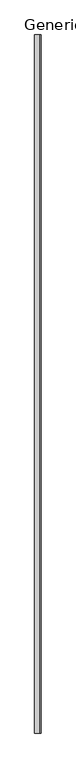
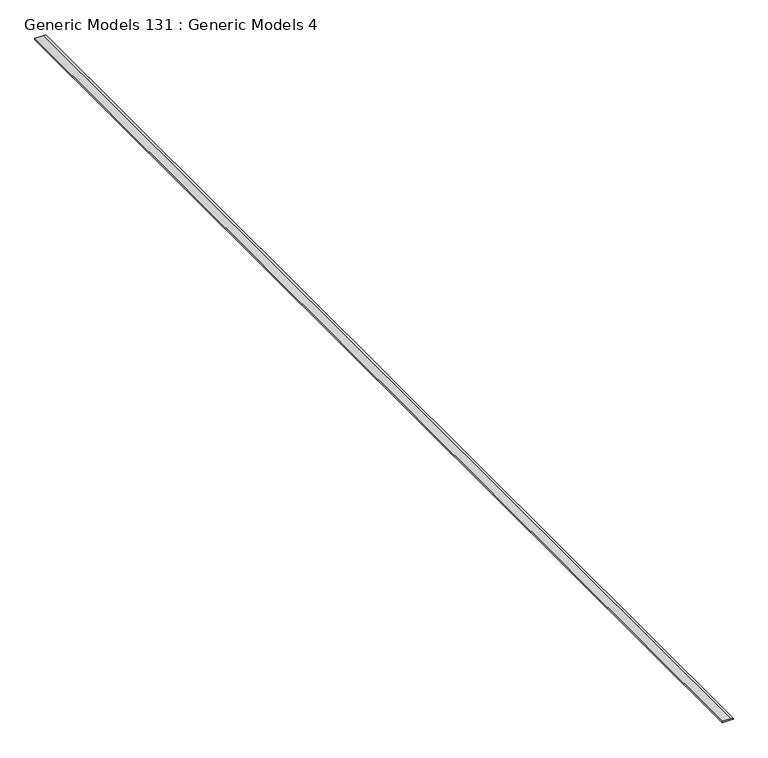
"""IFC4 building model written with IfcOpenShell, lengths in millimetres: proxy geometry, Generic Models 131 : Generic Models 4."""

import ifcopenshell
import ifcopenshell.guid

model = None  # the IFC model being written
_history = None  # IfcOwnerHistory: only IFC2X3 demands one
_inside = {}  # id of a spatial element -> (the spatial element, [elements in it])
_under = {}  # id of a project, library or spatial element -> (it, [spatial elements below it])
_declared = {}  # id of a project -> (the project, [libraries it declares])
_typed = {}  # id of a type object -> (the type object, [elements of that type])
_made_of = {}  # id of a material, layer set ... -> (it, [elements and type objects made of it])


def new_model(schema):
    """Start an empty IFC model of exactly this schema.

    Asked for "IFC4X3", IfcOpenShell would pick the latest addendum, in which some entities
    have other attributes; the version numbers below select the first issue.
    IFC2X3 requires an IfcOwnerHistory on every rooted entity: one is made here for all.
    """
    global model, _history
    if schema == "IFC4X3":
        model = ifcopenshell.file(schema_version=(4, 3, 0, 0))
    else:
        model = ifcopenshell.file(schema=schema)
    _inside.clear()
    _under.clear()
    _declared.clear()
    _typed.clear()
    _made_of.clear()
    _history = None
    if model.schema == "IFC2X3":
        org = make("IfcOrganization", Name="unknown")
        user = make(
            "IfcPersonAndOrganization",
            ThePerson=make("IfcPerson", FamilyName="unknown"),
            TheOrganization=org,
        )
        app = make(
            "IfcApplication",
            ApplicationDeveloper=org,
            Version="unknown",
            ApplicationFullName="unknown",
            ApplicationIdentifier="unknown",
        )
        _history = make(
            "IfcOwnerHistory",
            OwningUser=user,
            OwningApplication=app,
            ChangeAction="ADDED",
            CreationDate=0,
        )
    return model


def make(cls, **values):
    """One entity of the class cls with the attributes given. An attribute that is None is left unset."""
    return model.create_entity(
        cls, **{name: value for name, value in values.items() if value is not None}
    )


def rooted(cls, **values):
    """An entity with a GlobalId (a new one), such as an element, a storey or a relation."""
    return make(cls, GlobalId=ifcopenshell.guid.new(), OwnerHistory=_history, **values)


def si_unit(unit_type, name, prefix=None):
    """IfcSIUnit, for example si_unit("LENGTHUNIT", "METRE", prefix="MILLI")."""
    return make("IfcSIUnit", UnitType=unit_type, Prefix=prefix, Name=name)


def assignment(units):
    """IfcUnitAssignment: the units of a project."""
    return None if units is None else make("IfcUnitAssignment", Units=units)


def point(xyz):
    """IfcCartesianPoint."""
    return None if xyz is None else make("IfcCartesianPoint", Coordinates=xyz)


def direction(xyz):
    """IfcDirection."""
    return None if xyz is None else make("IfcDirection", DirectionRatios=xyz)


def frame(location, z_axis=None, x_axis=None):
    """IfcAxis2Placement3D, a coordinate frame: its origin and axes. An axis left out is left unset."""
    return make(
        "IfcAxis2Placement3D",
        Location=point(location),
        Axis=direction(z_axis),
        RefDirection=direction(x_axis),
    )


def origin():
    """The frame at (0, 0, 0) with its axes left unset."""
    return frame((0.0, 0.0, 0.0))


def place(relative_to, where):
    """IfcLocalPlacement: puts the frame where relative to a parent placement (None: the world)."""
    return make(
        "IfcLocalPlacement", PlacementRelTo=relative_to, RelativePlacement=where
    )


def context(
    kind, dimensions, precision=None, world=None, true_north=None, identifier=None
):
    """IfcGeometricRepresentationContext, for example the 3D "Model" context."""
    return make(
        "IfcGeometricRepresentationContext",
        ContextIdentifier=identifier,
        ContextType=kind,
        CoordinateSpaceDimension=dimensions,
        Precision=precision,
        WorldCoordinateSystem=world,
        TrueNorth=true_north,
    )


def project(units=None, contexts=None):
    """IfcProject with its units and contexts."""
    return rooted(
        "IfcProject",
        Name="project",
        RepresentationContexts=contexts,
        UnitsInContext=assignment(units),
    )


def spatial(cls, under=None, at=None, **own):
    """A site, building, storey or space (cls), placed at a placement, below another one or the project."""
    s = rooted(cls, ObjectPlacement=at, **own)
    if under is not None:
        _under.setdefault(under.id(), (under, []))[1].append(s)
    return s


def faces_of(points, faces, orient=None, outer=None):
    """IfcFace entities. A face is a list of loops; a loop is a list of indices into points, from 0.

    orient and outer hold one flag for each loop. By default every Orientation is true, the
    first loop of a face is its IfcFaceOuterBound and the others are IfcFaceBound.
    """
    made = []
    for i, loops in enumerate(faces):
        bounds = []
        for j, loop in enumerate(loops):
            is_outer = j == 0 if outer is None else outer[i][j]
            bounds.append(
                make(
                    "IfcFaceOuterBound" if is_outer else "IfcFaceBound",
                    Bound=make("IfcPolyLoop", Polygon=[points[k] for k in loop]),
                    Orientation=True if orient is None else orient[i][j],
                )
            )
        made.append(make("IfcFace", Bounds=bounds))
    return made


def faceted_brep(points, faces, orient=None, outer=None, voids=None):
    """IfcFacetedBrep: a solid bounded by flat faces; with voids (closed shells), ...WithVoids."""
    shared = [point(p) for p in points]
    hull = make("IfcClosedShell", CfsFaces=faces_of(shared, faces, orient, outer))
    if voids is None:
        return make("IfcFacetedBrep", Outer=hull)
    return make(
        "IfcFacetedBrepWithVoids",
        Outer=hull,
        Voids=[
            make(cls, CfsFaces=faces_of(shared, fs, o, b)) for cls, fs, o, b in voids
        ],
    )


def shape(context_of_items, identifier, shape_type, items):
    """IfcShapeRepresentation: the items that make up one representation, for example the "Body"."""
    return make(
        "IfcShapeRepresentation",
        ContextOfItems=context_of_items,
        RepresentationIdentifier=identifier,
        RepresentationType=shape_type,
        Items=items,
    )


def source(mapping_origin, context_of_items, identifier, shape_type, items):
    """IfcRepresentationMap: a shape defined once, which mapped items show again and again."""
    return make(
        "IfcRepresentationMap",
        MappingOrigin=mapping_origin,
        MappedRepresentation=shape(context_of_items, identifier, shape_type, items),
    )


def transform(
    local_origin,
    x_axis=None,
    y_axis=None,
    z_axis=None,
    scale=None,
    scale2=None,
    scale3=None,
    uniform=True,
):
    """IfcCartesianTransformationOperator3D, or its non-uniform kind. x_axis, y_axis, z_axis: its Axis1, 2, 3."""
    if uniform:
        return make(
            "IfcCartesianTransformationOperator3D",
            Axis1=direction(x_axis),
            Axis2=direction(y_axis),
            LocalOrigin=point(local_origin),
            Scale=scale,
            Axis3=direction(z_axis),
        )
    return make(
        "IfcCartesianTransformationOperator3DnonUniform",
        Axis1=direction(x_axis),
        Axis2=direction(y_axis),
        LocalOrigin=point(local_origin),
        Scale=scale,
        Axis3=direction(z_axis),
        Scale2=scale2,
        Scale3=scale3,
    )


def mapped(mapping_source, mapping_target):
    """IfcMappedItem: shows the shape of a source again, moved by a transform."""
    return make(
        "IfcMappedItem", MappingSource=mapping_source, MappingTarget=mapping_target
    )


def made_of(thing, what):
    """Note that an element or type object is made of a material, layer set ...; save() writes the relation."""
    if what is not None:
        _made_of.setdefault(what.id(), (what, []))[1].append(thing)
    return thing


def element(
    cls,
    number,
    at=None,
    inside=None,
    cuts=None,
    type_object=None,
    material=None,
    context=None,
    identifier="Body",
    shape_type=None,
    held_by="IfcProductDefinitionShape",
    body=None,
    shapes=None,
    **own,
):
    """One element of the class cls, such as IfcWall. Its Tag is "e" and its number.

    at: its placement. inside: the storey or other place that contains it. cuts: it is an
    opening in that element (IfcRelVoidsElement). A single representation is given by context,
    identifier, shape_type and body (its items); several are given by shapes. held_by: the class
    of the entity that holds the representations. save() writes the other relations.
    """
    e = rooted(cls, Tag="e%d" % number, ObjectPlacement=at, **own)
    if body is not None:
        shapes = [shape(context, identifier, shape_type, body)]
    if shapes is not None:
        e.Representation = make(held_by, Representations=shapes)
    if inside is not None:
        _inside.setdefault(inside.id(), (inside, []))[1].append(e)
    if cuts is not None:
        rooted(
            "IfcRelVoidsElement", RelatingBuildingElement=cuts, RelatedOpeningElement=e
        )
    if type_object is not None:
        _typed.setdefault(type_object.id(), (type_object, []))[1].append(e)
    return made_of(e, material)


def aggregate(whole, parts):
    """IfcRelAggregates: a whole, such as a stair, and the parts it consists of."""
    return rooted("IfcRelAggregates", RelatingObject=whole, RelatedObjects=parts)


def save(model, path):
    """Write the relations noted so far, then the file.

    IfcRelAggregates (storeys below a building ...), IfcRelContainedInSpatialStructure (elements
    in a storey), IfcRelDefinesByType, IfcRelAssociatesMaterial and IfcRelDeclares: one each for
    every whole, place, type object, material and project.
    """
    for whole, parts in _under.values():
        aggregate(whole, parts)
    for where, things in _inside.values():
        rooted(
            "IfcRelContainedInSpatialStructure",
            RelatedElements=things,
            RelatingStructure=where,
        )
    for kind, things in _typed.values():
        rooted("IfcRelDefinesByType", RelatedObjects=things, RelatingType=kind)
    for what, things in _made_of.values():
        rooted("IfcRelAssociatesMaterial", RelatedObjects=things, RelatingMaterial=what)
    for by, libraries in _declared.values():
        rooted("IfcRelDeclares", RelatingContext=by, RelatedDefinitions=libraries)
    model.write(path)


def generic_models_131_generic_models_4_27c2c8b5(model_context):
    return source(origin(), model_context, "Body", "Brep", [
        faceted_brep([(7087.6963704, -6864.9230338, 126305.691), (7110.1395544, -6864.9230338, 126305.691), (7110.1395544, -6864.9230338, 126304.421), (7250.4278204, -6864.9230338, 126304.421), (7250.4278204, -6864.9230338, 126307.4234564), (7251.6978204, -6864.9230338, 126307.4234564), (7251.6978204, -6864.9230338, 126305.691), (7253.9076204, -6864.9230338, 126305.691), (7253.9076204, -6864.9230338, 126325.376), (7217.0776204, -6864.9230338, 126325.376), (7217.0776204, -6864.9230338, 126326.646), (7087.6963704, -6864.9230338, 126326.646), (7087.6963704, -6864.9230338, 126317.121), (7110.1395544, 11778.6769662, 126305.691), (7087.6963704, 11778.6769662, 126305.691), (7087.6963704, 11778.6769662, 126317.121), (7087.6963704, 11778.6769662, 126326.646), (7217.0776204, 11778.6769662, 126326.646), (7217.0776204, 11778.6769662, 126325.376), (7253.9076204, 11778.6769662, 126325.376), (7253.9076204, 11778.6769662, 126305.691), (7251.6978204, 11778.6769662, 126305.691), (7251.6978204, 11778.6769662, 126307.4234564), (7250.4278204, 11778.6769662, 126307.4234564), (7250.4278204, 11778.6769662, 126304.421), (7110.1395544, 11778.6769662, 126304.421)], [[[0, 1, 2, 3, 4, 5, 6, 7, 8, 9, 10, 11, 12]], [[13, 14, 15, 16, 17, 18, 19, 20, 21, 22, 23, 24, 25]], [[16, 11, 10, 17]], [[2, 25, 24, 3]], [[11, 16, 15, 14, 0, 12]], [[8, 7, 20, 19]], [[9, 18, 17, 10]], [[18, 9, 8, 19]], [[6, 21, 20, 7]], [[4, 23, 22, 5]], [[23, 4, 3, 24]], [[21, 6, 5, 22]], [[25, 2, 1, 13]], [[1, 0, 14, 13]]]),
    ])


if __name__ == "__main__":
    model = new_model("IFC4")
    model_context = context("Model", 3, world=origin())
    ifc_project = project(units=[si_unit("LENGTHUNIT", "METRE", prefix="MILLI")], contexts=[model_context])
    site = spatial("IfcSite", under=ifc_project)
    building = spatial("IfcBuilding", under=site)
    placement = place(None, origin())
    generic_models_131_generic_models_4_shape = generic_models_131_generic_models_4_27c2c8b5(model_context)
    element("IfcBuildingElementProxy", 1, Name="Generic Models 131 : Generic Models 4", ObjectType="Generic Models 131 : Generic Models 4", at=placement, inside=building, context=model_context, shape_type="MappedRepresentation", body=[
        mapped(generic_models_131_generic_models_4_shape, transform((0.0, 0.0, 0.0), x_axis=(1.0, 0.0, 0.0), y_axis=(0.0, 1.0, 0.0), z_axis=(0.0, 0.0, 1.0))),
    ])
    save(model, "model.ifc")

# Revit data of these elements
# Element 1 (IfcBuildingElementProxy, "Generic Models 131 : Generic Models 4")
#   Materials on its faces: "_7/8\" SMOOTH TROWEL EXTERIOR STUCCO (COLOR PER OWNER)"
# Materials
#   "_7/8\" SMOOTH TROWEL EXTERIOR STUCCO (COLOR PER OWNER)": class "Generic", colour RGB 233 233 233, transparency 0, Cost = 0
